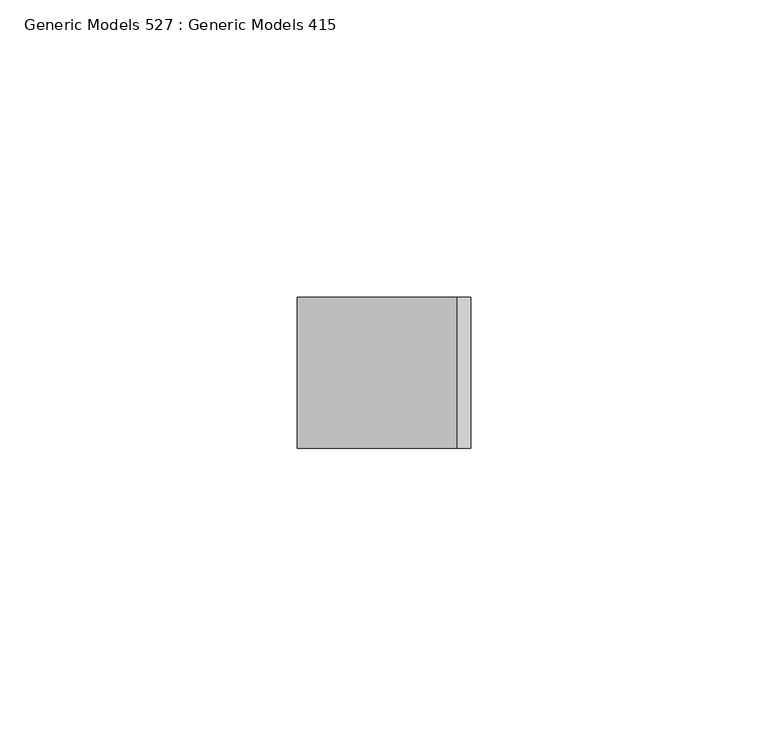
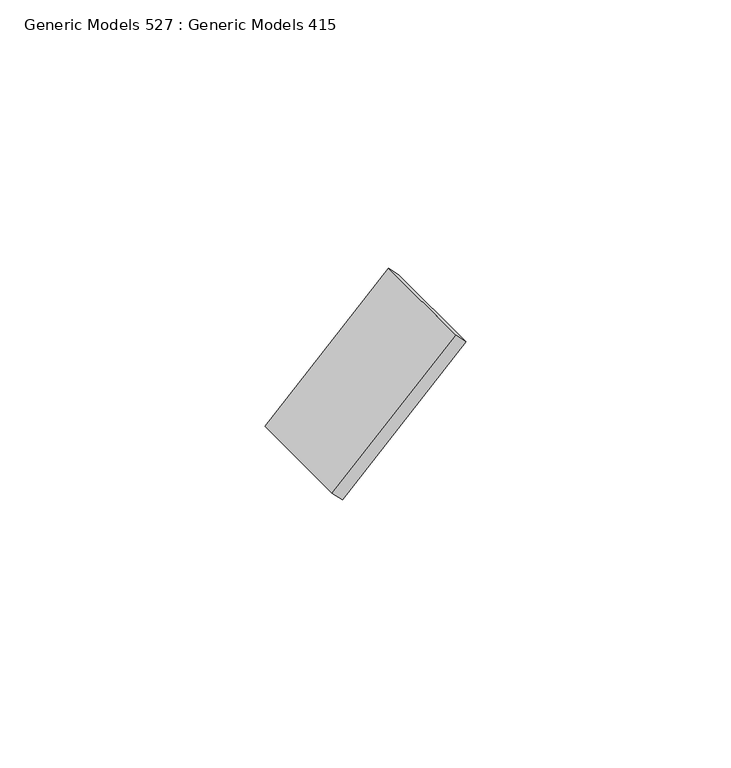
"""IFC4 building model written with IfcOpenShell, lengths in millimetres: proxy geometry, Generic Models 527 : Generic Models 415."""

import ifcopenshell
import ifcopenshell.guid

model = None  # the IFC model being written
_history = None  # IfcOwnerHistory: only IFC2X3 demands one
_inside = {}  # id of a spatial element -> (the spatial element, [elements in it])
_under = {}  # id of a project, library or spatial element -> (it, [spatial elements below it])
_declared = {}  # id of a project -> (the project, [libraries it declares])
_typed = {}  # id of a type object -> (the type object, [elements of that type])
_made_of = {}  # id of a material, layer set ... -> (it, [elements and type objects made of it])


def new_model(schema):
    """Start an empty IFC model of exactly this schema.

    Asked for "IFC4X3", IfcOpenShell would pick the latest addendum, in which some entities
    have other attributes; the version numbers below select the first issue.
    IFC2X3 requires an IfcOwnerHistory on every rooted entity: one is made here for all.
    """
    global model, _history
    if schema == "IFC4X3":
        model = ifcopenshell.file(schema_version=(4, 3, 0, 0))
    else:
        model = ifcopenshell.file(schema=schema)
    _inside.clear()
    _under.clear()
    _declared.clear()
    _typed.clear()
    _made_of.clear()
    _history = None
    if model.schema == "IFC2X3":
        org = make("IfcOrganization", Name="unknown")
        user = make(
            "IfcPersonAndOrganization",
            ThePerson=make("IfcPerson", FamilyName="unknown"),
            TheOrganization=org,
        )
        app = make(
            "IfcApplication",
            ApplicationDeveloper=org,
            Version="unknown",
            ApplicationFullName="unknown",
            ApplicationIdentifier="unknown",
        )
        _history = make(
            "IfcOwnerHistory",
            OwningUser=user,
            OwningApplication=app,
            ChangeAction="ADDED",
            CreationDate=0,
        )
    return model


def make(cls, **values):
    """One entity of the class cls with the attributes given. An attribute that is None is left unset."""
    return model.create_entity(
        cls, **{name: value for name, value in values.items() if value is not None}
    )


def rooted(cls, **values):
    """An entity with a GlobalId (a new one), such as an element, a storey or a relation."""
    return make(cls, GlobalId=ifcopenshell.guid.new(), OwnerHistory=_history, **values)


def si_unit(unit_type, name, prefix=None):
    """IfcSIUnit, for example si_unit("LENGTHUNIT", "METRE", prefix="MILLI")."""
    return make("IfcSIUnit", UnitType=unit_type, Prefix=prefix, Name=name)


def assignment(units):
    """IfcUnitAssignment: the units of a project."""
    return None if units is None else make("IfcUnitAssignment", Units=units)


def point(xyz):
    """IfcCartesianPoint."""
    return None if xyz is None else make("IfcCartesianPoint", Coordinates=xyz)


def direction(xyz):
    """IfcDirection."""
    return None if xyz is None else make("IfcDirection", DirectionRatios=xyz)


def frame(location, z_axis=None, x_axis=None):
    """IfcAxis2Placement3D, a coordinate frame: its origin and axes. An axis left out is left unset."""
    return make(
        "IfcAxis2Placement3D",
        Location=point(location),
        Axis=direction(z_axis),
        RefDirection=direction(x_axis),
    )


def origin():
    """The frame at (0, 0, 0) with its axes left unset."""
    return frame((0.0, 0.0, 0.0))


def place(relative_to, where):
    """IfcLocalPlacement: puts the frame where relative to a parent placement (None: the world)."""
    return make(
        "IfcLocalPlacement", PlacementRelTo=relative_to, RelativePlacement=where
    )


def context(
    kind, dimensions, precision=None, world=None, true_north=None, identifier=None
):
    """IfcGeometricRepresentationContext, for example the 3D "Model" context."""
    return make(
        "IfcGeometricRepresentationContext",
        ContextIdentifier=identifier,
        ContextType=kind,
        CoordinateSpaceDimension=dimensions,
        Precision=precision,
        WorldCoordinateSystem=world,
        TrueNorth=true_north,
    )


def project(units=None, contexts=None):
    """IfcProject with its units and contexts."""
    return rooted(
        "IfcProject",
        Name="project",
        RepresentationContexts=contexts,
        UnitsInContext=assignment(units),
    )


def spatial(cls, under=None, at=None, **own):
    """A site, building, storey or space (cls), placed at a placement, below another one or the project."""
    s = rooted(cls, ObjectPlacement=at, **own)
    if under is not None:
        _under.setdefault(under.id(), (under, []))[1].append(s)
    return s


def polyline(points):
    """IfcPolyline through the points."""
    return make("IfcPolyline", Points=[point(p) for p in points])


def outline(outer, holes=None, kind="AREA"):
    """IfcArbitraryClosedProfileDef: a profile drawn as a closed curve; with holes, ...WithVoids."""
    if holes is None:
        return make("IfcArbitraryClosedProfileDef", ProfileType=kind, OuterCurve=outer)
    return make(
        "IfcArbitraryProfileDefWithVoids",
        ProfileType=kind,
        OuterCurve=outer,
        InnerCurves=holes,
    )


def extrude(swept, where, along, depth):
    """IfcExtrudedAreaSolid: the profile swept, set in the frame where, extruded along a direction by depth."""
    return make(
        "IfcExtrudedAreaSolid",
        SweptArea=swept,
        Position=where,
        ExtrudedDirection=direction(along),
        Depth=depth,
    )


def shape(context_of_items, identifier, shape_type, items):
    """IfcShapeRepresentation: the items that make up one representation, for example the "Body"."""
    return make(
        "IfcShapeRepresentation",
        ContextOfItems=context_of_items,
        RepresentationIdentifier=identifier,
        RepresentationType=shape_type,
        Items=items,
    )


def source(mapping_origin, context_of_items, identifier, shape_type, items):
    """IfcRepresentationMap: a shape defined once, which mapped items show again and again."""
    return make(
        "IfcRepresentationMap",
        MappingOrigin=mapping_origin,
        MappedRepresentation=shape(context_of_items, identifier, shape_type, items),
    )


def transform(
    local_origin,
    x_axis=None,
    y_axis=None,
    z_axis=None,
    scale=None,
    scale2=None,
    scale3=None,
    uniform=True,
):
    """IfcCartesianTransformationOperator3D, or its non-uniform kind. x_axis, y_axis, z_axis: its Axis1, 2, 3."""
    if uniform:
        return make(
            "IfcCartesianTransformationOperator3D",
            Axis1=direction(x_axis),
            Axis2=direction(y_axis),
            LocalOrigin=point(local_origin),
            Scale=scale,
            Axis3=direction(z_axis),
        )
    return make(
        "IfcCartesianTransformationOperator3DnonUniform",
        Axis1=direction(x_axis),
        Axis2=direction(y_axis),
        LocalOrigin=point(local_origin),
        Scale=scale,
        Axis3=direction(z_axis),
        Scale2=scale2,
        Scale3=scale3,
    )


def mapped(mapping_source, mapping_target):
    """IfcMappedItem: shows the shape of a source again, moved by a transform."""
    return make(
        "IfcMappedItem", MappingSource=mapping_source, MappingTarget=mapping_target
    )


def made_of(thing, what):
    """Note that an element or type object is made of a material, layer set ...; save() writes the relation."""
    if what is not None:
        _made_of.setdefault(what.id(), (what, []))[1].append(thing)
    return thing


def element(
    cls,
    number,
    at=None,
    inside=None,
    cuts=None,
    type_object=None,
    material=None,
    context=None,
    identifier="Body",
    shape_type=None,
    held_by="IfcProductDefinitionShape",
    body=None,
    shapes=None,
    **own,
):
    """One element of the class cls, such as IfcWall. Its Tag is "e" and its number.

    at: its placement. inside: the storey or other place that contains it. cuts: it is an
    opening in that element (IfcRelVoidsElement). A single representation is given by context,
    identifier, shape_type and body (its items); several are given by shapes. held_by: the class
    of the entity that holds the representations. save() writes the other relations.
    """
    e = rooted(cls, Tag="e%d" % number, ObjectPlacement=at, **own)
    if body is not None:
        shapes = [shape(context, identifier, shape_type, body)]
    if shapes is not None:
        e.Representation = make(held_by, Representations=shapes)
    if inside is not None:
        _inside.setdefault(inside.id(), (inside, []))[1].append(e)
    if cuts is not None:
        rooted(
            "IfcRelVoidsElement", RelatingBuildingElement=cuts, RelatedOpeningElement=e
        )
    if type_object is not None:
        _typed.setdefault(type_object.id(), (type_object, []))[1].append(e)
    return made_of(e, material)


def aggregate(whole, parts):
    """IfcRelAggregates: a whole, such as a stair, and the parts it consists of."""
    return rooted("IfcRelAggregates", RelatingObject=whole, RelatedObjects=parts)


def save(model, path):
    """Write the relations noted so far, then the file.

    IfcRelAggregates (storeys below a building ...), IfcRelContainedInSpatialStructure (elements
    in a storey), IfcRelDefinesByType, IfcRelAssociatesMaterial and IfcRelDeclares: one each for
    every whole, place, type object, material and project.
    """
    for whole, parts in _under.values():
        aggregate(whole, parts)
    for where, things in _inside.values():
        rooted(
            "IfcRelContainedInSpatialStructure",
            RelatedElements=things,
            RelatingStructure=where,
        )
    for kind, things in _typed.values():
        rooted("IfcRelDefinesByType", RelatedObjects=things, RelatingType=kind)
    for what, things in _made_of.values():
        rooted("IfcRelAssociatesMaterial", RelatedObjects=things, RelatingMaterial=what)
    for by, libraries in _declared.values():
        rooted("IfcRelDeclares", RelatingContext=by, RelatedDefinitions=libraries)
    model.write(path)


def generic_models_527_generic_models_415_c37ad14f(model_context):
    return source(origin(), model_context, "Body", "SweptSolid", [
        extrude(outline(polyline([(0.0, -3.175), (0.0, 0.0), (25.4, 0.0), (25.4, -3.175), (0.0, -3.175)])), frame((7848.0411784, 4501.3863946, 125448.3849742), z_axis=(0.7071067811867181, 0.0, 0.707106781186377), x_axis=(0.0, -1.0, 0.0)), (0.0, 0.0, 1.0), 38.1),
    ])


if __name__ == "__main__":
    model = new_model("IFC4")
    model_context = context("Model", 3, world=origin())
    ifc_project = project(units=[si_unit("LENGTHUNIT", "METRE", prefix="MILLI")], contexts=[model_context])
    site = spatial("IfcSite", under=ifc_project)
    building = spatial("IfcBuilding", under=site)
    placement = place(None, origin())
    generic_models_527_generic_models_415_shape = generic_models_527_generic_models_415_c37ad14f(model_context)
    element("IfcBuildingElementProxy", 1, Name="Generic Models 527 : Generic Models 415", ObjectType="Generic Models 527 : Generic Models 415", at=placement, inside=building, context=model_context, shape_type="MappedRepresentation", body=[
        mapped(generic_models_527_generic_models_415_shape, transform((0.0, 0.0, 0.0), x_axis=(1.0, 0.0, 0.0), y_axis=(0.0, 1.0, 0.0), z_axis=(0.0, 0.0, 1.0))),
    ])
    save(model, "model.ifc")

# Revit data of these elements
# Element 1 (IfcBuildingElementProxy, "Generic Models 527 : Generic Models 415")
#   Materials on its faces: "_WELDED STEEL TABS FOR LOUVER ATTACHMENT"
# Materials
#   "_WELDED STEEL TABS FOR LOUVER ATTACHMENT": class "Metal", colour RGB 199 199 199, transparency 0, Description = "Structural steel 50ksi", Cost = 0
